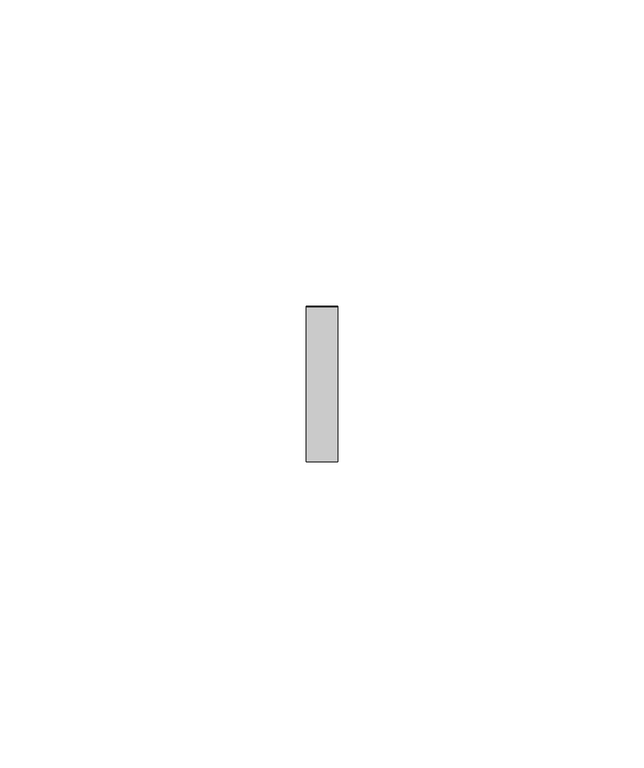
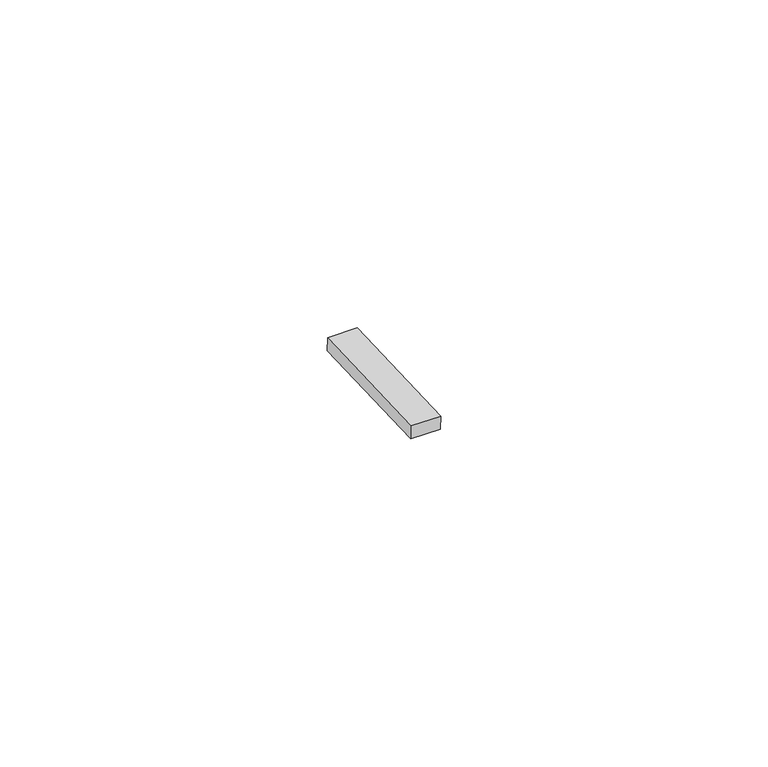
"""IFC4 building model written with IfcOpenShell, lengths in millimetres: proxy geometry, Inner panel:Inner panel:1:Inner panel:1 : Inner panel:Inner panel:300324:2:Inner panel:1:Inner panel:1 : Inner panel:Inner panel:300324:2 : Inner panel:Inner panel:1:Inner panel:1 : Inner panel:Inner panel:300324:300043:130 : Inner panel:Inner panel:1:Inner panel:1 : Inner panel:Inner panel:300324:2:Inner panel:1:Inner panel:1 : Inner panel:Inner panel:300324:2 : Inner panel:Inner panel:1:Inner panel:1 : Inner panel:Inner panel:300324:300043:308120."""

from ifc_helpers import new_model, si_unit, frame, origin, place, context, project, spatial, polyline, outline, extrude, source, transform, mapped, element, save


def generic_models_52f41098(model_context):
    return source(origin(), model_context, "Body", "SweptSolid", [
        extrude(outline(polyline([(0.0, -25.4), (0.0, 0.0), (5.2138089, 0.0), (5.2138089, -25.4), (0.0, -25.4)])), frame((593123.795117, -576574.3073926, 4050.9976844), z_axis=(0.0, -0.041630544712223896, 0.9991330730923502), x_axis=(-1.0, 0.0, 0.0)), (0.0, 0.0, 1.0), 2.4763745),
    ])


if __name__ == "__main__":
    model = new_model("IFC4")
    model_context = context("Model", 3, world=origin())
    ifc_project = project(units=[si_unit("LENGTHUNIT", "METRE", prefix="MILLI")], contexts=[model_context])
    site = spatial("IfcSite", under=ifc_project)
    building = spatial("IfcBuilding", under=site)
    placement = place(None, origin())
    generic_models_shape = generic_models_52f41098(model_context)
    element("IfcBuildingElementProxy", 1, Name="Inner panel:Inner panel:1:Inner panel:1 : Inner panel:Inner panel:300324:2:Inner panel:1:Inner panel:1 : Inner panel:Inner panel:300324:2 : Inner panel:Inner panel:1:Inner panel:1 : Inner panel:Inner panel:300324:300043:130 : Inner panel:Inner panel:1:Inner panel:1 : Inner panel:Inner panel:300324:2:Inner panel:1:Inner panel:1 : Inner panel:Inner panel:300324:2 : Inner panel:Inner panel:1:Inner panel:1 : Inner panel:Inner panel:300324:300043:308120", ObjectType="Inner panel:Inner panel:1:Inner panel:1 : Inner panel:Inner panel:300324:2:Inner panel:1:Inner panel:1 : Inner panel:Inner panel:300324:2 : Inner panel:Inner panel:1:Inner panel:1 : Inner panel:Inner panel:300324:300043:130 : Inner panel:Inner panel:1:Inner panel:1 : Inner panel:Inner panel:300324:2:Inner panel:1:Inner panel:1 : Inner panel:Inner panel:300324:2 : Inner panel:Inner panel:1:Inner panel:1 : Inner panel:Inner panel:300324:300043:308120", at=placement, inside=building, context=model_context, shape_type="MappedRepresentation", body=[
        mapped(generic_models_shape, transform((0.0, 0.0, 0.0), x_axis=(1.0, 0.0, 0.0), y_axis=(0.0, 1.0, 0.0), z_axis=(0.0, 0.0, 1.0))),
    ])
    save(model, "model.ifc")

# Revit data of these elements
# Type "Inner panel:Inner panel:1:Inner panel:1 : Inner panel:Inner panel:300324:2:Inner panel:1:Inner panel:1 : Inner panel:Inner panel:300324:2 : Inner panel:Inner panel:1:Inner panel:1 : Inner panel:Inner panel:300324:300043:130 : Inner panel:Inner panel:1:Inner panel:1 : Inner panel:Inner panel:300324:2:Inner panel:1:Inner panel:1 : Inner panel:Inner panel:300324:2 : Inner panel:Inner panel:1:Inner panel:1 : Inner panel:Inner panel:300324:300043:308120"
#   NameOverride = "Inner panel:Inner panel:1:Inner panel:1 : Inner panel:Inner panel:300324:2:Inner panel:1:Inner panel:1 : Inner panel:Inner panel:300324:2 : Inner panel:Inner panel:1:Inner panel:1 : Inner panel:Inner panel:300324:300043:308120"
#   ObjectTypeOverride = "Inner panel:1:Inner panel:1 : Inner panel:Inner panel:300324:2 : Inner panel:Inner panel:1:Inner panel:1 : Inner panel:Inner panel:300324:300043"
#   Reference = "Inner panel"
#   Tag = "308120"
# Element 1 (IfcBuildingElementProxy, "Inner panel:Inner panel:1:Inner panel:1 : Inner panel:Inner panel:300324:2:Inner panel:1:Inner panel:1 : Inner panel:Inner panel:300324:2 : Inner panel:Inner panel:1:Inner panel:1 : Inner panel:Inner panel:300324:300043:130 : Inner panel:Inner panel:1:Inner panel:1 : Inner panel:Inner panel:300324:2:Inner panel:1:Inner panel:1 : Inner panel:Inner panel:300324:2 : Inner panel:Inner panel:1:Inner panel:1 : Inner panel:Inner panel:300324:300043:308120")
#   Materials on its faces: "AT CLIP - 1\" WIDE NON ABSORBENT, WEATHER-RESISTANT NEOPRENE/EPDM/SBR FOAM"
# Materials
#   "AT CLIP - 1\" WIDE NON ABSORBENT, WEATHER-RESISTANT NEOPRENE/EPDM/SBR FOAM": class "Generic", colour RGB 85 85 85, transparency 0, Cost = 0
